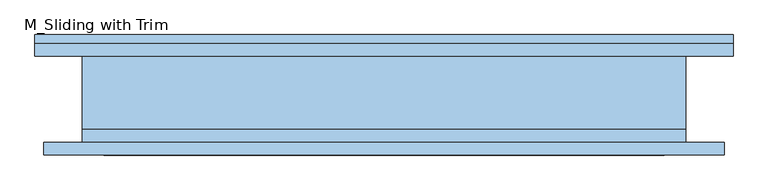
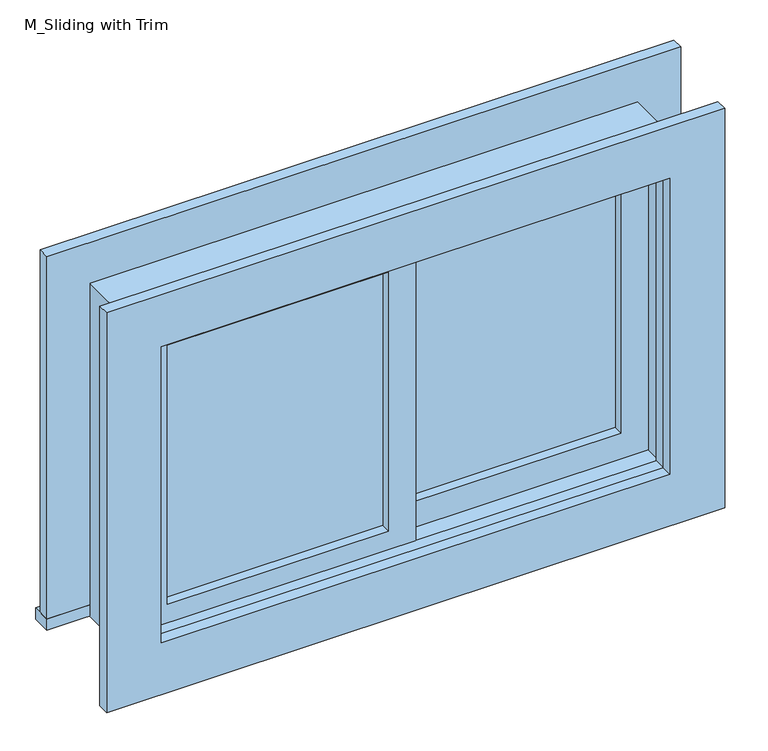
"""IFC4 building model written with IfcOpenShell, lengths in millimetres: window geometry, M_Sliding with Trim."""

from ifc_helpers import new_model, si_unit, frame, origin, place, context, project, spatial, polyline, outline, extrude, source, transform, mapped, element, save


def m_sliding_with_trim_861dbc4a(model_context):
    return source(origin(), model_context, "Body", "SweptSolid", [
        extrude(outline(polyline([(-381.0, -15.825), (-22.225, -15.825), (-22.225, -28.525), (-381.0, -28.525), (-381.0, -15.825)])), frame((0.0, 0.0, 1790.7), z_axis=(0.0, 0.0, 1.0), x_axis=(1.0, 0.0, 0.0)), (0.0, 0.0, 1.0), 444.5),
        extrude(outline(polyline([(2279.65, -425.45), (1746.25, -425.45), (1746.25, 22.225), (2279.65, 22.225), (2279.65, -425.45)]), holes=[polyline([(2235.2, -381.0), (2235.2, -22.225), (1790.7, -22.225), (1790.7, -381.0), (2235.2, -381.0)])]), frame((0.0, -44.4, 0.0), z_axis=(0.0, 1.0, 0.0), x_axis=(0.0, 0.0, 1.0)), (0.0, 0.0, 1.0), 44.45),
        extrude(outline(polyline([(-514.45, 95.2), (514.45, 95.2), (514.45, 63.5), (-514.45, 63.5), (-514.45, 95.2)])), frame((0.0, 0.0, 1727.2), z_axis=(0.0, 0.0, 1.0), x_axis=(1.0, 0.0, 0.0)), (0.0, 0.0, 1.0), 19.05),
        extrude(outline(polyline([(2279.65, -425.45), (2279.65, 425.45), (1746.25, 425.45), (1746.25, 514.45), (2368.65, 514.45), (2368.65, -514.45), (1746.25, -514.45), (1746.25, -425.45), (2279.65, -425.45)])), frame((0.0, 63.5, 0.0), z_axis=(0.0, 1.0, 0.0), x_axis=(0.0, 0.0, 1.0)), (0.0, 0.0, 1.0), 19.0),
        extrude(outline(polyline([(2355.95, 501.75), (2355.95, -501.75), (1669.95, -501.75), (1669.95, 501.75), (2355.95, 501.75)]), holes=[polyline([(2266.95, 412.75), (1758.95, 412.75), (1758.95, -412.75), (2266.95, -412.75), (2266.95, 412.75)])]), frame((0.0, -82.5, 0.0), z_axis=(0.0, 1.0, 0.0), x_axis=(0.0, 0.0, 1.0)), (0.0, 0.0, 1.0), 19.0),
        extrude(outline(polyline([(381.0, 15.925), (22.225, 15.925), (22.225, 28.625), (381.0, 28.625), (381.0, 15.925)])), frame((0.0, 0.0, 1790.7), z_axis=(0.0, 0.0, 1.0), x_axis=(1.0, 0.0, 0.0)), (0.0, 0.0, 1.0), 444.5),
        extrude(outline(polyline([(2279.65, -22.225), (1746.25, -22.225), (1746.25, 425.45), (2279.65, 425.45), (2279.65, -22.225)]), holes=[polyline([(2235.2, 22.225), (2235.2, 381.0), (1790.7, 381.0), (1790.7, 22.225), (2235.2, 22.225)])]), frame((0.0, 0.05, 0.0), z_axis=(0.0, 1.0, 0.0), x_axis=(0.0, 0.0, 1.0)), (0.0, 0.0, 1.0), 44.45),
        extrude(outline(polyline([(2298.7, -444.5), (1727.2, -444.5), (1727.2, 444.5), (2298.7, 444.5), (2298.7, -444.5)]), holes=[polyline([(2266.95, -412.75), (2266.95, 412.75), (1758.95, 412.75), (1758.95, -412.75), (2266.95, -412.75)])]), frame((0.0, -63.5, 0.0), z_axis=(0.0, 1.0, 0.0), x_axis=(0.0, 0.0, 1.0)), (0.0, 0.0, 1.0), 19.1),
        extrude(outline(polyline([(2298.7, 444.5), (2298.7, -444.5), (1727.2, -444.5), (1727.2, 444.5), (2298.7, 444.5)]), holes=[polyline([(2279.65, 425.45), (1746.25, 425.45), (1746.25, -425.45), (2279.65, -425.45), (2279.65, 425.45)])]), frame((0.0, -44.4, 0.0), z_axis=(0.0, 1.0, 0.0), x_axis=(0.0, 0.0, 1.0)), (0.0, 0.0, 1.0), 107.9),
    ])


if __name__ == "__main__":
    model = new_model("IFC4")
    model_context = context("Model", 3, world=origin())
    ifc_project = project(units=[si_unit("LENGTHUNIT", "METRE", prefix="MILLI")], contexts=[model_context])
    site = spatial("IfcSite", under=ifc_project)
    building = spatial("IfcBuilding", under=site)
    placement = place(None, origin())
    m_sliding_with_trim_shape = m_sliding_with_trim_861dbc4a(model_context)
    element("IfcWindow", 1, ObjectType="M_Sliding with Trim : 2'  11\" x 1'  10 1/2\" @ 5'  8\"", at=placement, inside=building, context=model_context, shape_type="MappedRepresentation", body=[
        mapped(m_sliding_with_trim_shape, transform((0.0, 0.0, 0.0), x_axis=(1.0, 0.0, 0.0), y_axis=(0.0, 1.0, 0.0), z_axis=(0.0, 0.0, 1.0))),
    ])
    save(model, "model.ifc")

# Revit data of these elements
# Type "M_Sliding with Trim : 2'  11\" x 1'  10 1/2\" @ 5'  8\""
#   Type Mark = "66"
#   Construction Type Id = "GSP4R"
#   Analytic Construction = "1/8 in Pilkington single glazing"
#   Visual Light Transmittance = 0.9
#   Solar Heat Gain Coefficient = 0.78
#   Heat Transfer Coefficient (U) = 3.6886 W/(m²·K)
#   Height = 1' - 10 1/2"
#   Default Sill Height = 5' - 8"
#   Trim Projection - Ext. = 0' - 0.74803"
#   Trim Projection - Int. = 0' - 0.74803"
#   Trim Width - Exterior = 0' - 3.50394"
#   Trim Width - Interior = 0' - 3.50394"
#   Width = 2' - 11"
#   Window Inset = 0' - 0.74803"
#   Glass Pane Material = EXISTING WINDOW
#   Sash Material = Trim
#   Trim Exterior Material = Trim
#   Trim Interior Material = Trim
#   Wall Closure = (empty or 0)
# Element 1 (IfcWindow, "M_Sliding with Trim : 2'  11\" x 1'  10 1/2\" @ 5'  8\"")
#   Materials on its faces: "Trim", "EXISTING WINDOW"
# Materials
#   "EXISTING WINDOW": class "Glass", colour RGB 218 227 224, transparency 0.85, Description = "Soda Lime Glass", Cost = 0
#   "Trim": class "Wood", colour RGB 250 251 245, transparency 0, Cost = 0
